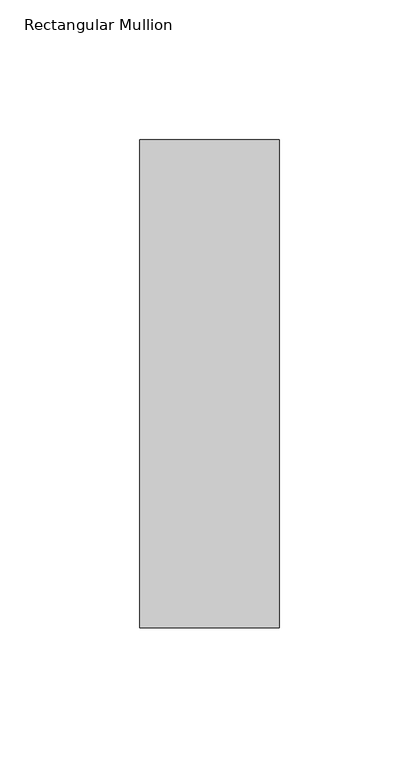
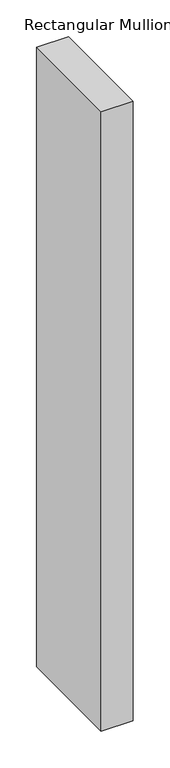
"""IFC4 building model written with IfcOpenShell, lengths in millimetres: member geometry, Rectangular Mullion : WWm-50x175-50mmOffset."""

from ifc_helpers import new_model, si_unit, frame, origin, place, context, project, spatial, polyline, outline, extrude, source, transform, mapped, element, save


def rectangular_mullion_3ec656f4(model_context):
    return source(origin(), model_context, "Body", "SweptSolid", [
        extrude(outline(polyline([(0.0, 87.5), (0.0, -87.5), (-50.0, -87.5), (-50.0, 87.5), (0.0, 87.5)])), frame((0.0, 0.0, -1025.0), z_axis=(0.0, 0.0, 1.0), x_axis=(1.0, 0.0, 0.0)), (0.0, 0.0, 1.0), 1025.0),
    ])


if __name__ == "__main__":
    model = new_model("IFC4")
    model_context = context("Model", 3, world=origin())
    ifc_project = project(units=[si_unit("LENGTHUNIT", "METRE", prefix="MILLI")], contexts=[model_context])
    site = spatial("IfcSite", under=ifc_project)
    building = spatial("IfcBuilding", under=site)
    placement = place(None, origin())
    rectangular_mullion_shape = rectangular_mullion_3ec656f4(model_context)
    element("IfcMember", 1, ObjectType="Rectangular Mullion : WWm-50x175-50mmOffset", at=placement, inside=building, context=model_context, shape_type="MappedRepresentation", body=[
        mapped(rectangular_mullion_shape, transform((0.0, 0.0, 0.0), x_axis=(1.0, 0.0, 0.0), y_axis=(0.0, 1.0, 0.0), z_axis=(0.0, 0.0, 1.0))),
    ])
    save(model, "model.ifc")

# Revit data of these elements
# Type "Rectangular Mullion : WWm-50x175-50mmOffset"
#   built-in parameter 1007304 = 0.574147 (stored number, unit not read)
#   built-in parameter 1007301 = 0.082021 (stored number, unit not read)
#   built-in parameter 1007300 = 0.082021 (stored number, unit not read)
# Element 1 (IfcMember, "Rectangular Mullion : WWm-50x175-50mmOffset")
#   Materials on its faces: "WW-EC-RGB-Mullion"
# Materials
#   "WW-EC-RGB-Mullion": class "Generic", colour RGB 255 255 255, transparency 0, Comments = "If region requests black mullions, switch asset color to RGB 25-25-25", Description = "Generic Color", Cost = 0
